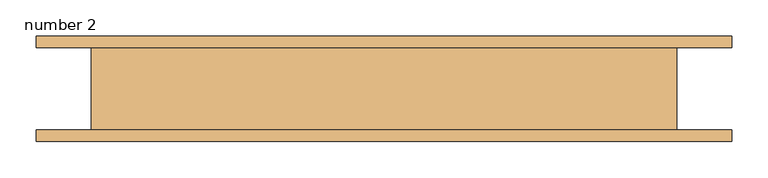
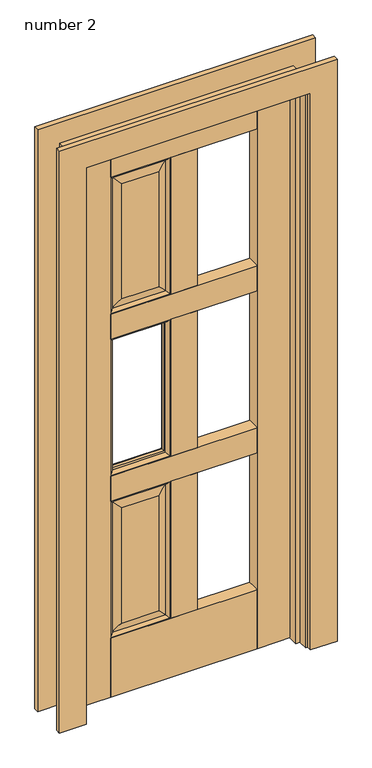
"""IFC4 building model written with IfcOpenShell, lengths in millimetres: door geometry, Door-Interior-Karona-K5660-6_Panel : number 2."""

from ifc_helpers import new_model, si_unit, frame, origin, origin_with_axes, place, context, project, spatial, polyline, ellipse_curve, outline, extrude, faceted_brep, source, transform, mapped, element, save
from ifc_brep_helpers import plane_surface, cylinder_surface, revolved_surface, advanced_brep


def number_2_7843cb6c(model_context):
    return source(origin(), model_context, "Body", "SolidModel", [
        advanced_brep(
        [(-254.0, 15.2908, 1311.275), (-242.6746863, 24.6126, 1299.9496863), (-57.3628137, 24.6126, 1299.9496863), (-46.0375, 15.2908, 1311.275), (-57.1627, 46.3324899, 1300.1498), (-48.2727, 54.4576, 1309.0398), (-48.2727, 54.4576, 811.8602), (-57.1627, 46.3324899, 820.7502), (-242.8748, 46.3324899, 820.7502), (-251.7648, 54.4576, 811.8602), (-251.7648, 54.4576, 1309.0398), (-242.8748, 46.3324899, 1300.1498), (-46.0375, 54.4576, 809.625), (-46.0375, 15.2908, 809.625), (-254.0, 15.2908, 809.625), (-254.0, 54.4576, 809.625), (-57.1627, 34.7218, 820.7502), (-242.8748, 34.7218, 820.7502), (-47.3075, 24.6126, 1310.005), (-47.3075, 34.7218, 1310.005), (-47.3075, 34.7218, 810.895), (-47.3075, 24.6126, 810.895), (-252.73, 24.6126, 810.895), (-252.73, 24.6126, 1310.005), (-57.3628137, 24.6126, 820.9503137), (-242.6746863, 24.6126, 820.9503137), (-252.73, 34.7218, 810.895), (-254.0, 54.4576, 1311.275), (-242.8748, 34.7218, 1300.1498), (-252.73, 34.7218, 1310.005), (-46.0375, 54.4576, 1311.275), (-57.1627, 34.7218, 1300.1498)],
        [
            (0, 1, ellipse_curve(frame((-252.9689876, 25.5788135, 1310.2439876), z_axis=(0.7071067811865475, 0.0, 0.7071067811865475), x_axis=(-0.7071067811865476, 0.0, 0.7071067811865474)), 14.6223259, 10.3395458)),
            (1, 2),
            (2, 3, ellipse_curve(frame((-47.0685124, 25.5788135, 1310.2439876), z_axis=(-0.7071067811865475, 0.0, 0.7071067811865475), x_axis=(-0.7071067811865476, 0.0, -0.7071067811865474)), 14.6223259, 10.3395458)),
            (3, 0),
            (4, 5, ellipse_curve(frame((-48.2727, 45.531597, 1309.0398), z_axis=(0.7071067811865475, 0.0, -0.7071067811865475), x_axis=(0.7071067811865474, 0.0, 0.7071067811865476)), 12.6232745, 8.926003)),
            (5, 6),
            (6, 7, ellipse_curve(frame((-48.2727, 45.531597, 811.8602), z_axis=(0.7071067811865475, 0.0, 0.7071067811865475), x_axis=(-0.7071067811865474, 0.0, 0.7071067811865476)), 12.6232745, 8.926003)),
            (7, 4),
            (8, 9, ellipse_curve(frame((-251.7648, 45.531597, 811.8602), z_axis=(-0.7071067811865475, 0.0, 0.7071067811865475), x_axis=(-0.7071067811865474, 0.0, -0.7071067811865476)), 12.6232745, 8.926003)),
            (9, 10),
            (10, 11, ellipse_curve(frame((-251.7648, 45.531597, 1309.0398), z_axis=(-0.7071067811865475, 0.0, -0.7071067811865475), x_axis=(0.7071067811865474, 0.0, -0.7071067811865476)), 12.6232745, 8.926003)),
            (11, 8),
            (12, 13),
            (13, 14),
            (14, 15),
            (15, 12),
            (16, 7),
            (7, 8),
            (8, 17),
            (17, 16),
            (18, 19),
            (19, 20),
            (20, 21),
            (21, 18),
            (22, 23),
            (23, 18),
            (21, 22),
            (24, 2),
            (1, 25),
            (25, 24),
            (13, 24, ellipse_curve(frame((-47.0685124, 25.5788135, 810.6560124), z_axis=(-0.7071067811865475, 0.0, -0.7071067811865475), x_axis=(0.7071067811865476, 0.0, -0.7071067811865474)), 14.6223259, 10.3395458)),
            (25, 14, ellipse_curve(frame((-252.9689876, 25.5788135, 810.6560124), z_axis=(0.7071067811865475, 0.0, -0.7071067811865475), x_axis=(0.7071067811865476, 0.0, 0.7071067811865474)), 14.6223259, 10.3395458)),
            (20, 26),
            (26, 22),
            (14, 0),
            (0, 27),
            (27, 15),
            (11, 28),
            (28, 17),
            (26, 29),
            (29, 23),
            (3, 30),
            (30, 27),
            (11, 4),
            (4, 31),
            (31, 28),
            (29, 19),
            (3, 13),
            (12, 30),
            (16, 31),
            (5, 10),
            (9, 6),
        ],
        [
            cylinder_surface(frame((-254.0, 25.5788135, 1310.2439876), z_axis=(-1.0, 0.0, 0.0), x_axis=(0.0, -1.0, 0.0)), 10.3395458),
            cylinder_surface(frame((-48.2727, 45.531597, 1311.275), z_axis=(0.0, 0.0, 1.0), x_axis=(0.0, -1.0, 0.0)), 8.926003),
            cylinder_surface(frame((-251.7648, 45.531597, 809.625), z_axis=(0.0, 0.0, -1.0), x_axis=(0.0, -1.0, 0.0)), 8.926003),
            plane_surface(frame((-46.0375, 15.2908, 809.625), z_axis=(0.0, 0.0, -1.0), x_axis=(-1.0, 0.0, 0.0))),
            plane_surface(frame((-57.1627, 46.3324899, 820.7502), z_axis=(0.0, 0.0, 1.0), x_axis=(-1.0, 0.0, 0.0))),
            plane_surface(frame((-47.3075, 34.7218, 1310.005), z_axis=(-1.0, 0.0, 0.0), x_axis=(0.0, 0.0, -1.0))),
            plane_surface(frame((-47.3075, 24.6126, 1310.005), z_axis=(0.0, 1.0, 0.0), x_axis=(0.0, 0.0, -1.0))),
            cylinder_surface(frame((-46.0375, 25.5788135, 810.6560124), z_axis=(1.0, 0.0, 0.0), x_axis=(0.0, -1.0, 0.0)), 10.3395458),
            plane_surface(frame((-47.3075, 34.7218, 810.895), z_axis=(0.0, 0.0, 1.0), x_axis=(-1.0, 0.0, 0.0))),
            plane_surface(frame((-254.0, 15.2908, 809.625), z_axis=(-1.0, 0.0, 0.0), x_axis=(0.0, 0.0, 1.0))),
            plane_surface(frame((-242.8748, 46.3324899, 820.7502), z_axis=(1.0, 0.0, 0.0), x_axis=(0.0, 0.0, 1.0))),
            plane_surface(frame((-252.73, 34.7218, 810.895), z_axis=(1.0, 0.0, 0.0), x_axis=(0.0, 0.0, 1.0))),
            plane_surface(frame((-254.0, 15.2908, 1311.275), z_axis=(0.0, 0.0, 1.0), x_axis=(1.0, 0.0, 0.0))),
            plane_surface(frame((-242.8748, 46.3324899, 1300.1498), z_axis=(0.0, 0.0, -1.0), x_axis=(1.0, 0.0, 0.0))),
            plane_surface(frame((-252.73, 34.7218, 1310.005), z_axis=(0.0, 0.0, -1.0), x_axis=(1.0, 0.0, 0.0))),
            plane_surface(frame((-46.0375, 15.2908, 1311.275), z_axis=(1.0, 0.0, 0.0), x_axis=(0.0, 0.0, -1.0))),
            plane_surface(frame((-57.1627, 46.3324899, 1300.1498), z_axis=(-1.0, 0.0, 0.0), x_axis=(0.0, 0.0, -1.0))),
            plane_surface(frame((-57.1627, 34.7218, 1300.1498), z_axis=(0.0, -1.0, 0.0), x_axis=(0.0, 0.0, -1.0))),
            plane_surface(frame((-46.0375, 54.4576, 1311.275), z_axis=(0.0, 1.0, 0.0), x_axis=(0.0, 0.0, -1.0))),
            cylinder_surface(frame((-46.0375, 45.531597, 811.8602), z_axis=(1.0, 0.0, 0.0), x_axis=(0.0, -1.0, 0.0)), 8.926003),
            cylinder_surface(frame((-252.9689876, 25.5788135, 809.625), z_axis=(0.0, 0.0, -1.0), x_axis=(0.0, -1.0, 0.0)), 10.3395458),
            cylinder_surface(frame((-254.0, 45.531597, 1309.0398), z_axis=(-1.0, 0.0, 0.0), x_axis=(0.0, -1.0, 0.0)), 8.926003),
            cylinder_surface(frame((-47.0685124, 25.5788135, 1311.275), z_axis=(0.0, 0.0, 1.0), x_axis=(0.0, -1.0, 0.0)), 10.3395458),
        ],
        [
            (0, [[1, 2, 3, 4]]),
            (1, [[5, 6, 7, 8]]),
            (2, [[9, 10, 11, 12]]),
            (3, [[13, 14, 15, 16]]),
            (4, [[17, 18, 19, 20]]),
            (5, [[21, 22, 23, 24]]),
            (6, [[25, 26, -24, 27], [28, -2, 29, 30]]),
            (7, [[31, -30, 32, -14]]),
            (8, [[-23, 33, 34, -27]]),
            (9, [[-15, 35, 36, 37]]),
            (10, [[-19, -12, 38, 39]]),
            (11, [[-34, 40, 41, -25]]),
            (12, [[-36, -4, 42, 43]]),
            (13, [[-38, 44, 45, 46]]),
            (14, [[-41, 47, -21, -26]]),
            (15, [[-42, 48, -13, 49]]),
            (16, [[-45, -8, -17, 50]]),
            (17, [[-22, -47, -40, -33], [-39, -46, -50, -20]]),
            (18, [[-37, -43, -49, -16], [-6, 51, -10, 52]]),
            (19, [[-7, -52, -9, -18]]),
            (20, [[-32, -29, -1, -35]]),
            (21, [[-11, -51, -5, -44]]),
            (22, [[-3, -28, -31, -48]]),
        ],
    ),
        advanced_brep(
        [(-242.8748, 54.4576, 1893.8748), (-57.1627, 54.4576, 1893.8748), (-57.1627, 54.4576, 1414.4752), (-242.8748, 54.4576, 1414.4752), (-242.8748, 34.7218, 1893.8748), (-57.1627, 34.7218, 1893.8748), (-57.1627, 36.0454899, 1893.8748), (-242.8748, 36.0454899, 1893.8748), (-242.8748, 44.5515929, 1893.8748), (-57.1627, 44.5515929, 1893.8748), (-57.1627, 34.7218, 1414.4752), (-242.8748, 34.7218, 1414.4752), (-242.8748, 36.0454899, 1414.4752), (-57.1627, 36.0454899, 1414.4752), (-57.1627, 44.5515929, 1414.4752), (-242.8748, 44.5515929, 1414.4752), (-87.1686653, 44.5515929, 1863.8688347), (-212.8688347, 44.5515929, 1863.8688347), (-87.1686653, 44.5515929, 1444.4811653), (-212.8688347, 44.5515929, 1444.4811653)],
        [
            (0, 1),
            (1, 2),
            (2, 3),
            (3, 0),
            (4, 5),
            (5, 6),
            (6, 7),
            (7, 4),
            (0, 8),
            (8, 9),
            (9, 1),
            (10, 11),
            (11, 12),
            (12, 13),
            (13, 10),
            (2, 14),
            (14, 15),
            (15, 3),
            (15, 8),
            (11, 4),
            (7, 12),
            (9, 14),
            (5, 10),
            (13, 6),
            (16, 17),
            (17, 7, ellipse_curve(frame((-244.8131685, 100.0605261, 1895.8131685), z_axis=(-0.7071067811865475, 0.0, -0.7071067811865475), x_axis=(-0.7071067811865476, 0.0, 0.7071067811865474)), 90.5724254, 64.0443762)),
            (6, 16, ellipse_curve(frame((-55.2243315, 100.0605261, 1895.8131685), z_axis=(0.7071067811865475, 0.0, -0.7071067811865475), x_axis=(-0.7071067811865476, 0.0, -0.7071067811865474)), 90.5724254, 64.0443762)),
            (18, 16),
            (13, 18, ellipse_curve(frame((-55.2243315, 100.0605261, 1412.5368315), z_axis=(-0.7071067811865475, 0.0, -0.7071067811865475), x_axis=(-0.7071067811865474, 0.0, 0.7071067811865476)), 90.5724254, 64.0443762)),
            (19, 18),
            (12, 19, ellipse_curve(frame((-244.8131685, 100.0605261, 1412.5368315), z_axis=(-0.7071067811865475, 0.0, 0.7071067811865475), x_axis=(0.7071067811865476, 0.0, 0.7071067811865474)), 90.5724254, 64.0443762)),
            (17, 19),
        ],
        [
            plane_surface(frame((-57.1627, 54.4576, 1893.8748), z_axis=(0.0, 1.0, 0.0), x_axis=(0.0, 0.0, -1.0))),
            plane_surface(frame((-57.1627, 34.7218, 1893.8748), z_axis=(0.0, 0.0, 1.0), x_axis=(1.0, 0.0, 0.0))),
            plane_surface(frame((-57.1627, 34.7218, 1414.4752), z_axis=(0.0, 0.0, -1.0), x_axis=(-1.0, 0.0, 0.0))),
            plane_surface(frame((-242.8748, 54.4576, 1893.8748), z_axis=(-1.0, 0.0, 0.0), x_axis=(0.0, 0.0, -1.0))),
            plane_surface(frame((-57.1627, 34.7218, 1893.8748), z_axis=(1.0, 0.0, 0.0), x_axis=(0.0, 0.0, -1.0))),
            plane_surface(frame((-242.8748, 34.7218, 1893.8748), z_axis=(0.0, -1.0, 0.0), x_axis=(0.0, 0.0, -1.0))),
            revolved_surface(polyline([(-308.8575446888527, 100.0605261, 1831.7687923), (8.820044688852704, 100.0605261, 1831.7687923)]), (-254.0, 100.0605261, 1895.8131685), (-1.0, 0.0, 0.0)),
            revolved_surface(polyline([(-119.2687077, 100.0605261, 1959.8575446888528), (-119.2687077, 100.0605261, 1348.4924553111473)]), (-55.2243315, 100.0605261, 1905.0), (0.0, 0.0, 1.0)),
            revolved_surface(polyline([(8.820044688852683, 100.0605261, 1476.5812077), (-308.8575446888527, 100.0605261, 1476.5812077)]), (-46.0375, 100.0605261, 1412.5368315), (1.0, 0.0, 0.0)),
            revolved_surface(polyline([(-180.76879229999997, 100.0605261, 1348.4924553111473), (-180.76879229999997, 100.0605261, 1959.8575446888526)]), (-244.8131685, 100.0605261, 1403.35), (0.0, 0.0, -1.0)),
            plane_surface(frame((-254.0, 44.5515929, 1403.35), z_axis=(0.0, -1.0, 0.0), x_axis=(0.0, 0.0, 1.0))),
        ],
        [
            (0, [[1, 2, 3, 4]]),
            (1, [[5, 6, 7, 8]]),
            (1, [[-1, 9, 10, 11]]),
            (2, [[12, 13, 14, 15]]),
            (2, [[-3, 16, 17, 18]]),
            (3, [[-4, -18, 19, -9]]),
            (3, [[20, -8, 21, -13]]),
            (4, [[-2, -11, 22, -16]]),
            (4, [[23, -15, 24, -6]]),
            (5, [[-5, -20, -12, -23]]),
            (6, [[25, 26, -7, 27]]),
            (7, [[28, -27, -24, 29]]),
            (8, [[30, -29, -14, 31]]),
            (9, [[32, -31, -21, -26]]),
            (10, [[-10, -19, -17, -22], [-25, -28, -30, -32]]),
        ],
    ),
        advanced_brep(
        [(-242.8748, 24.6126, 1893.8748), (-57.1627, 24.6126, 1893.8748), (-57.1627, 24.6126, 1414.4752), (-242.8748, 24.6126, 1414.4752), (-214.0448579, 15.4432, 1443.3051421), (-85.9926421, 15.4432, 1443.3051421), (-85.9926421, 15.4432, 1865.0448579), (-214.0448579, 15.4432, 1865.0448579), (-242.8748, 23.2889101, 1893.8748), (-57.1627, 23.2889101, 1893.8748), (-57.1627, 23.2889101, 1414.4752), (-242.8748, 23.2889101, 1414.4752)],
        [
            (0, 1),
            (1, 2),
            (2, 3),
            (3, 0),
            (4, 5),
            (5, 6),
            (6, 7),
            (7, 4),
            (0, 8),
            (8, 9),
            (9, 1),
            (2, 10),
            (10, 11),
            (11, 3),
            (4, 11, ellipse_curve(frame((-244.8131685, -40.7261261, 1412.5368315), z_axis=(-0.7071067811865475, 0.0, 0.7071067811865475), x_axis=(0.7071067811865476, 0.0, 0.7071067811865474)), 90.5724254, 64.0443762)),
            (10, 5, ellipse_curve(frame((-55.2243315, -40.7261261, 1412.5368315), z_axis=(0.7071067811865475, 0.0, 0.7071067811865475), x_axis=(0.7071067811865476, 0.0, -0.7071067811865474)), 90.5724254, 64.0443762)),
            (7, 8, ellipse_curve(frame((-244.8131685, -40.7261261, 1895.8131685), z_axis=(0.7071067811865475, 0.0, 0.7071067811865475), x_axis=(0.7071067811865474, 0.0, -0.7071067811865476)), 90.5724254, 64.0443762)),
            (8, 11),
            (6, 9, ellipse_curve(frame((-55.2243315, -40.7261261, 1895.8131685), z_axis=(0.7071067811865475, 0.0, -0.7071067811865475), x_axis=(-0.7071067811865476, 0.0, -0.7071067811865474)), 90.5724254, 64.0443762)),
            (10, 9),
        ],
        [
            plane_surface(frame((-57.1627, 24.6126, 1893.8748), z_axis=(0.0, 1.0, 0.0), x_axis=(0.0, 0.0, -1.0))),
            plane_surface(frame((-242.8748, 15.4432, 1893.8748), z_axis=(0.0, -1.0, 0.0), x_axis=(0.0, 0.0, -1.0))),
            plane_surface(frame((-57.1627, 34.7218, 1893.8748), z_axis=(0.0, 0.0, 1.0), x_axis=(1.0, 0.0, 0.0))),
            plane_surface(frame((-57.1627, 34.7218, 1414.4752), z_axis=(0.0, 0.0, -1.0), x_axis=(-1.0, 0.0, 0.0))),
            revolved_surface(polyline([(8.820044688852711, -40.7261261, 1476.5812077), (-308.8575446888527, -40.7261261, 1476.5812077)]), (-46.0375, -40.7261261, 1412.5368315), (1.0, 0.0, 0.0)),
            revolved_surface(polyline([(-180.76879229999997, -40.7261261, 1348.4924553111473), (-180.76879229999997, -40.7261261, 1959.8575446888528)]), (-244.8131685, -40.7261261, 1403.35), (0.0, 0.0, -1.0)),
            revolved_surface(polyline([(-308.85754468885267, -40.7261261, 1831.7687923), (8.820044688852704, -40.7261261, 1831.7687923)]), (-254.0, -40.7261261, 1895.8131685), (-1.0, 0.0, 0.0)),
            revolved_surface(polyline([(-119.2687077, -40.7261261, 1959.8575446888528), (-119.2687077, -40.7261261, 1348.4924553111473)]), (-55.2243315, -40.7261261, 1905.0), (0.0, 0.0, 1.0)),
            plane_surface(frame((-242.8748, 24.6126, 1893.8748), z_axis=(-1.0, 0.0, 0.0), x_axis=(0.0, 0.0, -1.0))),
            plane_surface(frame((-57.1627, 15.4432, 1893.8748), z_axis=(1.0, 0.0, 0.0), x_axis=(0.0, 0.0, -1.0))),
        ],
        [
            (0, [[1, 2, 3, 4]]),
            (1, [[5, 6, 7, 8]]),
            (2, [[-1, 9, 10, 11]]),
            (3, [[-3, 12, 13, 14]]),
            (4, [[15, -13, 16, -5]]),
            (5, [[-15, -8, 17, 18]]),
            (6, [[-17, -7, 19, -10]]),
            (7, [[-19, -6, -16, 20]]),
            (8, [[-4, -14, -18, -9]]),
            (9, [[-2, -11, -20, -12]]),
        ],
    ),
        advanced_brep(
        [(-254.0, 15.2908, 1905.0), (-242.6746863, 24.6126, 1893.6746863), (-57.3628137, 24.6126, 1893.6746863), (-46.0375, 15.2908, 1905.0), (-57.1627, 46.3324899, 1893.8748), (-48.2727, 54.4576, 1902.7648), (-48.2727, 54.4576, 1405.5852), (-57.1627, 46.3324899, 1414.4752), (-242.8748, 46.3324899, 1414.4752), (-251.7648, 54.4576, 1405.5852), (-251.7648, 54.4576, 1902.7648), (-242.8748, 46.3324899, 1893.8748), (-46.0375, 54.4576, 1403.35), (-46.0375, 15.2908, 1403.35), (-254.0, 15.2908, 1403.35), (-254.0, 54.4576, 1403.35), (-57.1627, 34.7218, 1414.4752), (-242.8748, 34.7218, 1414.4752), (-47.3075, 24.6126, 1903.73), (-47.3075, 34.7218, 1903.73), (-47.3075, 34.7218, 1404.62), (-47.3075, 24.6126, 1404.62), (-252.73, 24.6126, 1404.62), (-252.73, 24.6126, 1903.73), (-57.3628137, 24.6126, 1414.6753137), (-242.6746863, 24.6126, 1414.6753137), (-252.73, 34.7218, 1404.62), (-254.0, 54.4576, 1905.0), (-242.8748, 34.7218, 1893.8748), (-252.73, 34.7218, 1903.73), (-46.0375, 54.4576, 1905.0), (-57.1627, 34.7218, 1893.8748)],
        [
            (0, 1, ellipse_curve(frame((-252.9689876, 25.5788135, 1903.9689876), z_axis=(0.7071067811865475, 0.0, 0.7071067811865475), x_axis=(-0.7071067811865476, 0.0, 0.7071067811865474)), 14.6223259, 10.3395458)),
            (1, 2),
            (2, 3, ellipse_curve(frame((-47.0685124, 25.5788135, 1903.9689876), z_axis=(-0.7071067811865475, 0.0, 0.7071067811865475), x_axis=(-0.7071067811865476, 0.0, -0.7071067811865474)), 14.6223259, 10.3395458)),
            (3, 0),
            (4, 5, ellipse_curve(frame((-48.2727, 45.531597, 1902.7648), z_axis=(0.7071067811865475, 0.0, -0.7071067811865475), x_axis=(0.7071067811865474, 0.0, 0.7071067811865476)), 12.6232745, 8.926003)),
            (5, 6),
            (6, 7, ellipse_curve(frame((-48.2727, 45.531597, 1405.5852), z_axis=(0.7071067811865475, 0.0, 0.7071067811865475), x_axis=(-0.7071067811865474, 0.0, 0.7071067811865476)), 12.6232745, 8.926003)),
            (7, 4),
            (8, 9, ellipse_curve(frame((-251.7648, 45.531597, 1405.5852), z_axis=(-0.7071067811865475, 0.0, 0.7071067811865475), x_axis=(-0.7071067811865474, 0.0, -0.7071067811865476)), 12.6232745, 8.926003)),
            (9, 10),
            (10, 11, ellipse_curve(frame((-251.7648, 45.531597, 1902.7648), z_axis=(-0.7071067811865475, 0.0, -0.7071067811865475), x_axis=(0.7071067811865474, 0.0, -0.7071067811865476)), 12.6232745, 8.926003)),
            (11, 8),
            (12, 13),
            (13, 14),
            (14, 15),
            (15, 12),
            (16, 7),
            (7, 8),
            (8, 17),
            (17, 16),
            (18, 19),
            (19, 20),
            (20, 21),
            (21, 18),
            (22, 23),
            (23, 18),
            (21, 22),
            (24, 2),
            (1, 25),
            (25, 24),
            (13, 24, ellipse_curve(frame((-47.0685124, 25.5788135, 1404.3810124), z_axis=(-0.7071067811865475, 0.0, -0.7071067811865475), x_axis=(0.7071067811865476, 0.0, -0.7071067811865474)), 14.6223259, 10.3395458)),
            (25, 14, ellipse_curve(frame((-252.9689876, 25.5788135, 1404.3810124), z_axis=(0.7071067811865475, 0.0, -0.7071067811865475), x_axis=(0.7071067811865476, 0.0, 0.7071067811865474)), 14.6223259, 10.3395458)),
            (20, 26),
            (26, 22),
            (14, 0),
            (0, 27),
            (27, 15),
            (11, 28),
            (28, 17),
            (26, 29),
            (29, 23),
            (3, 30),
            (30, 27),
            (11, 4),
            (4, 31),
            (31, 28),
            (29, 19),
            (3, 13),
            (12, 30),
            (16, 31),
            (5, 10),
            (9, 6),
        ],
        [
            cylinder_surface(frame((-254.0, 25.5788135, 1903.9689876), z_axis=(-1.0, 0.0, 0.0), x_axis=(0.0, -1.0, 0.0)), 10.3395458),
            cylinder_surface(frame((-48.2727, 45.531597, 1905.0), z_axis=(0.0, 0.0, 1.0), x_axis=(0.0, -1.0, 0.0)), 8.926003),
            cylinder_surface(frame((-251.7648, 45.531597, 1403.35), z_axis=(0.0, 0.0, -1.0), x_axis=(0.0, -1.0, 0.0)), 8.926003),
            plane_surface(frame((-46.0375, 15.2908, 1403.35), z_axis=(0.0, 0.0, -1.0), x_axis=(-1.0, 0.0, 0.0))),
            plane_surface(frame((-57.1627, 46.3324899, 1414.4752), z_axis=(0.0, 0.0, 1.0), x_axis=(-1.0, 0.0, 0.0))),
            plane_surface(frame((-47.3075, 34.7218, 1903.73), z_axis=(-1.0, 0.0, 0.0), x_axis=(0.0, 0.0, -1.0))),
            plane_surface(frame((-47.3075, 24.6126, 1903.73), z_axis=(0.0, 1.0, 0.0), x_axis=(0.0, 0.0, -1.0))),
            cylinder_surface(frame((-46.0375, 25.5788135, 1404.3810124), z_axis=(1.0, 0.0, 0.0), x_axis=(0.0, -1.0, 0.0)), 10.3395458),
            plane_surface(frame((-47.3075, 34.7218, 1404.62), z_axis=(0.0, 0.0, 1.0), x_axis=(-1.0, 0.0, 0.0))),
            plane_surface(frame((-254.0, 15.2908, 1403.35), z_axis=(-1.0, 0.0, 0.0), x_axis=(0.0, 0.0, 1.0))),
            plane_surface(frame((-242.8748, 46.3324899, 1414.4752), z_axis=(1.0, 0.0, 0.0), x_axis=(0.0, 0.0, 1.0))),
            plane_surface(frame((-252.73, 34.7218, 1404.62), z_axis=(1.0, 0.0, 0.0), x_axis=(0.0, 0.0, 1.0))),
            plane_surface(frame((-254.0, 15.2908, 1905.0), z_axis=(0.0, 0.0, 1.0), x_axis=(1.0, 0.0, 0.0))),
            plane_surface(frame((-242.8748, 46.3324899, 1893.8748), z_axis=(0.0, 0.0, -1.0), x_axis=(1.0, 0.0, 0.0))),
            plane_surface(frame((-252.73, 34.7218, 1903.73), z_axis=(0.0, 0.0, -1.0), x_axis=(1.0, 0.0, 0.0))),
            plane_surface(frame((-46.0375, 15.2908, 1905.0), z_axis=(1.0, 0.0, 0.0), x_axis=(0.0, 0.0, -1.0))),
            plane_surface(frame((-57.1627, 46.3324899, 1893.8748), z_axis=(-1.0, 0.0, 0.0), x_axis=(0.0, 0.0, -1.0))),
            plane_surface(frame((-57.1627, 34.7218, 1893.8748), z_axis=(0.0, -1.0, 0.0), x_axis=(0.0, 0.0, -1.0))),
            plane_surface(frame((-46.0375, 54.4576, 1905.0), z_axis=(0.0, 1.0, 0.0), x_axis=(0.0, 0.0, -1.0))),
            cylinder_surface(frame((-46.0375, 45.531597, 1405.5852), z_axis=(1.0, 0.0, 0.0), x_axis=(0.0, -1.0, 0.0)), 8.926003),
            cylinder_surface(frame((-252.9689876, 25.5788135, 1403.35), z_axis=(0.0, 0.0, -1.0), x_axis=(0.0, -1.0, 0.0)), 10.3395458),
            cylinder_surface(frame((-254.0, 45.531597, 1902.7648), z_axis=(-1.0, 0.0, 0.0), x_axis=(0.0, -1.0, 0.0)), 8.926003),
            cylinder_surface(frame((-47.0685124, 25.5788135, 1905.0), z_axis=(0.0, 0.0, 1.0), x_axis=(0.0, -1.0, 0.0)), 10.3395458),
        ],
        [
            (0, [[1, 2, 3, 4]]),
            (1, [[5, 6, 7, 8]]),
            (2, [[9, 10, 11, 12]]),
            (3, [[13, 14, 15, 16]]),
            (4, [[17, 18, 19, 20]]),
            (5, [[21, 22, 23, 24]]),
            (6, [[25, 26, -24, 27], [28, -2, 29, 30]]),
            (7, [[31, -30, 32, -14]]),
            (8, [[-23, 33, 34, -27]]),
            (9, [[-15, 35, 36, 37]]),
            (10, [[-19, -12, 38, 39]]),
            (11, [[-34, 40, 41, -25]]),
            (12, [[-36, -4, 42, 43]]),
            (13, [[-38, 44, 45, 46]]),
            (14, [[-41, 47, -21, -26]]),
            (15, [[-42, 48, -13, 49]]),
            (16, [[-45, -8, -17, 50]]),
            (17, [[-22, -47, -40, -33], [-39, -46, -50, -20]]),
            (18, [[-37, -43, -49, -16], [-6, 51, -10, 52]]),
            (19, [[-7, -52, -9, -18]]),
            (20, [[-32, -29, -1, -35]]),
            (21, [[-11, -51, -5, -44]]),
            (22, [[-3, -28, -31, -48]]),
        ],
    ),
        advanced_brep(
        [(-242.8748, 34.7218, 706.4248), (-57.1627, 34.7218, 706.4248), (-57.1627, 36.0454899, 706.4248), (-242.8748, 36.0454899, 706.4248), (-57.1627, 54.4576, 706.4248), (-242.8748, 54.4576, 706.4248), (-242.8748, 44.5515929, 706.4248), (-57.1627, 44.5515929, 706.4248), (-57.1627, 34.7218, 227.0252), (-242.8748, 34.7218, 227.0252), (-242.8748, 36.0454899, 227.0252), (-57.1627, 36.0454899, 227.0252), (-242.8748, 54.4576, 227.0252), (-57.1627, 54.4576, 227.0252), (-57.1627, 44.5515929, 227.0252), (-242.8748, 44.5515929, 227.0252), (-87.1686653, 44.5515929, 676.4188347), (-212.8688347, 44.5515929, 676.4188347), (-87.1686653, 44.5515929, 257.0311653), (-212.8688347, 44.5515929, 257.0311653)],
        [
            (0, 1),
            (1, 2),
            (2, 3),
            (3, 0),
            (4, 5),
            (5, 6),
            (6, 7),
            (7, 4),
            (8, 9),
            (9, 10),
            (10, 11),
            (11, 8),
            (12, 13),
            (13, 14),
            (14, 15),
            (15, 12),
            (5, 12),
            (15, 6),
            (9, 0),
            (3, 10),
            (4, 13),
            (7, 14),
            (1, 8),
            (11, 2),
            (16, 17),
            (17, 3, ellipse_curve(frame((-244.8131685, 100.0605261, 708.3631685), z_axis=(-0.7071067811865475, 0.0, -0.7071067811865475), x_axis=(-0.7071067811865476, 0.0, 0.7071067811865474)), 90.5724254, 64.0443762)),
            (2, 16, ellipse_curve(frame((-55.2243315, 100.0605261, 708.3631685), z_axis=(0.7071067811865475, 0.0, -0.7071067811865475), x_axis=(-0.7071067811865476, 0.0, -0.7071067811865474)), 90.5724254, 64.0443762)),
            (18, 16),
            (11, 18, ellipse_curve(frame((-55.2243315, 100.0605261, 225.0868315), z_axis=(-0.7071067811865475, 0.0, -0.7071067811865475), x_axis=(-0.7071067811865474, 0.0, 0.7071067811865476)), 90.5724254, 64.0443762)),
            (19, 18),
            (10, 19, ellipse_curve(frame((-244.8131685, 100.0605261, 225.0868315), z_axis=(-0.7071067811865475, 0.0, 0.7071067811865475), x_axis=(0.7071067811865476, 0.0, 0.7071067811865474)), 90.5724254, 64.0443762)),
            (17, 19),
        ],
        [
            plane_surface(frame((-57.1627, 34.7218, 706.4248), z_axis=(0.0, 0.0, 1.0), x_axis=(1.0, 0.0, 0.0))),
            plane_surface(frame((-57.1627, 34.7218, 227.0252), z_axis=(0.0, 0.0, -1.0), x_axis=(-1.0, 0.0, 0.0))),
            plane_surface(frame((-242.8748, 54.4576, 706.4248), z_axis=(-1.0, 0.0, 0.0), x_axis=(0.0, 0.0, -1.0))),
            plane_surface(frame((-57.1627, 54.4576, 706.4248), z_axis=(0.0, 1.0, 0.0), x_axis=(0.0, 0.0, -1.0))),
            plane_surface(frame((-57.1627, 34.7218, 706.4248), z_axis=(1.0, 0.0, 0.0), x_axis=(0.0, 0.0, -1.0))),
            plane_surface(frame((-242.8748, 34.7218, 706.4248), z_axis=(0.0, -1.0, 0.0), x_axis=(0.0, 0.0, -1.0))),
            revolved_surface(polyline([(-308.8575446888527, 100.0605261, 644.3187923), (8.820044688852704, 100.0605261, 644.3187923)]), (-254.0, 100.0605261, 708.3631685), (-1.0, 0.0, 0.0)),
            revolved_surface(polyline([(-119.2687077, 100.0605261, 772.4075446888527), (-119.2687077, 100.0605261, 161.04245531114725)]), (-55.2243315, 100.0605261, 717.55), (0.0, 0.0, 1.0)),
            revolved_surface(polyline([(8.820044688852683, 100.0605261, 289.1312077), (-308.8575446888527, 100.0605261, 289.1312077)]), (-46.0375, 100.0605261, 225.0868315), (1.0, 0.0, 0.0)),
            revolved_surface(polyline([(-180.76879229999997, 100.0605261, 161.0424553111473), (-180.76879229999997, 100.0605261, 772.4075446888527)]), (-244.8131685, 100.0605261, 215.9), (0.0, 0.0, -1.0)),
            plane_surface(frame((-254.0, 44.5515929, 215.9), z_axis=(0.0, -1.0, 0.0), x_axis=(0.0, 0.0, 1.0))),
        ],
        [
            (0, [[1, 2, 3, 4]]),
            (0, [[5, 6, 7, 8]]),
            (1, [[9, 10, 11, 12]]),
            (1, [[13, 14, 15, 16]]),
            (2, [[17, -16, 18, -6]]),
            (2, [[19, -4, 20, -10]]),
            (3, [[-5, 21, -13, -17]]),
            (4, [[-21, -8, 22, -14]]),
            (4, [[23, -12, 24, -2]]),
            (5, [[-1, -19, -9, -23]]),
            (6, [[25, 26, -3, 27]]),
            (7, [[28, -27, -24, 29]]),
            (8, [[30, -29, -11, 31]]),
            (9, [[32, -31, -20, -26]]),
            (10, [[-7, -18, -15, -22], [-25, -28, -30, -32]]),
        ],
    ),
        advanced_brep(
        [(-57.1627, 24.6126, 706.4248), (-242.8748, 24.6126, 706.4248), (-242.8748, 23.2889101, 706.4248), (-57.1627, 23.2889101, 706.4248), (-242.8748, 24.6126, 227.0252), (-57.1627, 24.6126, 227.0252), (-57.1627, 23.2889101, 227.0252), (-242.8748, 23.2889101, 227.0252), (-214.0448579, 15.4432, 255.8551421), (-85.9926421, 15.4432, 255.8551421), (-85.9926421, 15.4432, 677.5948579), (-214.0448579, 15.4432, 677.5948579)],
        [
            (0, 1),
            (1, 2),
            (2, 3),
            (3, 0),
            (4, 5),
            (5, 6),
            (6, 7),
            (7, 4),
            (0, 5),
            (4, 1),
            (8, 9),
            (9, 10),
            (10, 11),
            (11, 8),
            (8, 7, ellipse_curve(frame((-244.8131685, -40.7261261, 225.0868315), z_axis=(-0.7071067811865475, 0.0, 0.7071067811865475), x_axis=(0.7071067811865476, 0.0, 0.7071067811865474)), 90.5724254, 64.0443762)),
            (6, 9, ellipse_curve(frame((-55.2243315, -40.7261261, 225.0868315), z_axis=(0.7071067811865475, 0.0, 0.7071067811865475), x_axis=(0.7071067811865476, 0.0, -0.7071067811865474)), 90.5724254, 64.0443762)),
            (11, 2, ellipse_curve(frame((-244.8131685, -40.7261261, 708.3631685), z_axis=(0.7071067811865475, 0.0, 0.7071067811865475), x_axis=(0.7071067811865474, 0.0, -0.7071067811865476)), 90.5724254, 64.0443762)),
            (2, 7),
            (10, 3, ellipse_curve(frame((-55.2243315, -40.7261261, 708.3631685), z_axis=(0.7071067811865475, 0.0, -0.7071067811865475), x_axis=(-0.7071067811865476, 0.0, -0.7071067811865474)), 90.5724254, 64.0443762)),
            (6, 3),
        ],
        [
            plane_surface(frame((-57.1627, 34.7218, 706.4248), z_axis=(0.0, 0.0, 1.0), x_axis=(1.0, 0.0, 0.0))),
            plane_surface(frame((-57.1627, 34.7218, 227.0252), z_axis=(0.0, 0.0, -1.0), x_axis=(-1.0, 0.0, 0.0))),
            plane_surface(frame((-57.1627, 24.6126, 706.4248), z_axis=(0.0, 1.0, 0.0), x_axis=(0.0, 0.0, -1.0))),
            plane_surface(frame((-242.8748, 15.4432, 706.4248), z_axis=(0.0, -1.0, 0.0), x_axis=(0.0, 0.0, -1.0))),
            revolved_surface(polyline([(8.820044688852711, -40.7261261, 289.1312077), (-308.8575446888527, -40.7261261, 289.1312077)]), (-46.0375, -40.7261261, 225.0868315), (1.0, 0.0, 0.0)),
            revolved_surface(polyline([(-180.76879229999997, -40.7261261, 161.0424553111473), (-180.76879229999997, -40.7261261, 772.4075446888527)]), (-244.8131685, -40.7261261, 215.9), (0.0, 0.0, -1.0)),
            revolved_surface(polyline([(-308.85754468885267, -40.7261261, 644.3187923), (8.820044688852704, -40.7261261, 644.3187923)]), (-254.0, -40.7261261, 708.3631685), (-1.0, 0.0, 0.0)),
            revolved_surface(polyline([(-119.2687077, -40.7261261, 772.4075446888527), (-119.2687077, -40.7261261, 161.04245531114736)]), (-55.2243315, -40.7261261, 717.55), (0.0, 0.0, 1.0)),
            plane_surface(frame((-242.8748, 24.6126, 706.4248), z_axis=(-1.0, 0.0, 0.0), x_axis=(0.0, 0.0, -1.0))),
            plane_surface(frame((-57.1627, 15.4432, 706.4248), z_axis=(1.0, 0.0, 0.0), x_axis=(0.0, 0.0, -1.0))),
        ],
        [
            (0, [[1, 2, 3, 4]]),
            (1, [[5, 6, 7, 8]]),
            (2, [[-1, 9, -5, 10]]),
            (3, [[11, 12, 13, 14]]),
            (4, [[15, -7, 16, -11]]),
            (5, [[-15, -14, 17, 18]]),
            (6, [[-17, -13, 19, -3]]),
            (7, [[-19, -12, -16, 20]]),
            (8, [[-10, -8, -18, -2]]),
            (9, [[-9, -4, -20, -6]]),
        ],
    ),
        advanced_brep(
        [(-254.0, 15.2908, 717.55), (-242.6746863, 24.6126, 706.2246863), (-57.3628137, 24.6126, 706.2246863), (-46.0375, 15.2908, 717.55), (-57.1627, 46.3324899, 706.4248), (-48.2727, 54.4576, 715.3148), (-48.2727, 54.4576, 218.1352), (-57.1627, 46.3324899, 227.0252), (-254.0, 54.4576, 215.9), (-254.0, 54.4576, 717.55), (-46.0375, 54.4576, 717.55), (-46.0375, 54.4576, 215.9), (-251.7648, 54.4576, 715.3148), (-251.7648, 54.4576, 218.1352), (-46.0375, 15.2908, 215.9), (-254.0, 15.2908, 215.9), (-57.1627, 34.7218, 227.0252), (-242.8748, 46.3324899, 227.0252), (-242.8748, 34.7218, 227.0252), (-47.3075, 24.6126, 217.17), (-47.3075, 34.7218, 217.17), (-252.73, 34.7218, 217.17), (-252.73, 24.6126, 217.17), (-242.8748, 46.3324899, 706.4248), (-242.8748, 34.7218, 706.4248), (-252.73, 34.7218, 716.28), (-252.73, 24.6126, 716.28), (-57.1627, 34.7218, 706.4248), (-47.3075, 34.7218, 716.28), (-47.3075, 24.6126, 716.28), (-57.3628137, 24.6126, 227.2253137), (-242.6746863, 24.6126, 227.2253137)],
        [
            (0, 1, ellipse_curve(frame((-252.9689876, 25.5788135, 716.5189876), z_axis=(0.7071067811865475, 0.0, 0.7071067811865475), x_axis=(-0.7071067811865476, 0.0, 0.7071067811865474)), 14.6223259, 10.3395458)),
            (1, 2),
            (2, 3, ellipse_curve(frame((-47.0685124, 25.5788135, 716.5189876), z_axis=(-0.7071067811865475, 0.0, 0.7071067811865475), x_axis=(-0.7071067811865476, 0.0, -0.7071067811865474)), 14.6223259, 10.3395458)),
            (3, 0),
            (4, 5, ellipse_curve(frame((-48.2727, 45.531597, 715.3148), z_axis=(0.7071067811865475, 0.0, -0.7071067811865475), x_axis=(0.7071067811865474, 0.0, 0.7071067811865476)), 12.6232745, 8.926003)),
            (5, 6),
            (6, 7, ellipse_curve(frame((-48.2727, 45.531597, 218.1352), z_axis=(0.7071067811865475, 0.0, 0.7071067811865475), x_axis=(-0.7071067811865474, 0.0, 0.7071067811865476)), 12.6232745, 8.926003)),
            (7, 4),
            (8, 9),
            (9, 10),
            (10, 11),
            (11, 8),
            (5, 12),
            (12, 13),
            (13, 6),
            (11, 14),
            (14, 15),
            (15, 8),
            (16, 7),
            (7, 17),
            (17, 18),
            (18, 16),
            (19, 20),
            (20, 21),
            (21, 22),
            (22, 19),
            (15, 0),
            (0, 9),
            (17, 23),
            (23, 24),
            (24, 18),
            (21, 25),
            (25, 26),
            (26, 22),
            (3, 10),
            (23, 4),
            (4, 27),
            (27, 24),
            (25, 28),
            (28, 29),
            (29, 26),
            (3, 14),
            (16, 27),
            (20, 28),
            (19, 29),
            (30, 2),
            (1, 31),
            (31, 30),
            (30, 14, ellipse_curve(frame((-47.0685124, 25.5788135, 216.9310124), z_axis=(0.7071067811865475, 0.0, 0.7071067811865475), x_axis=(-0.7071067811865474, 0.0, 0.7071067811865476)), 14.6223259, 10.3395458)),
            (17, 13, ellipse_curve(frame((-251.7648, 45.531597, 218.1352), z_axis=(-0.7071067811865475, 0.0, 0.7071067811865475), x_axis=(-0.7071067811865474, 0.0, -0.7071067811865476)), 12.6232745, 8.926003)),
            (12, 23, ellipse_curve(frame((-251.7648, 45.531597, 715.3148), z_axis=(-0.7071067811865475, 0.0, -0.7071067811865475), x_axis=(0.7071067811865474, 0.0, -0.7071067811865476)), 12.6232745, 8.926003)),
            (31, 15, ellipse_curve(frame((-252.9689876, 25.5788135, 216.9310124), z_axis=(0.7071067811865475, 0.0, -0.7071067811865475), x_axis=(0.7071067811865476, 0.0, 0.7071067811865474)), 14.6223259, 10.3395458)),
        ],
        [
            cylinder_surface(frame((-254.0, 25.5788135, 716.5189876), z_axis=(-1.0, 0.0, 0.0), x_axis=(0.0, -1.0, 0.0)), 10.3395458),
            cylinder_surface(frame((-48.2727, 45.531597, 717.55), z_axis=(0.0, 0.0, 1.0), x_axis=(0.0, -1.0, 0.0)), 8.926003),
            plane_surface(frame((-46.0375, 54.4576, 717.55), z_axis=(0.0, 1.0, 0.0), x_axis=(0.0, 0.0, -1.0))),
            plane_surface(frame((-46.0375, 15.2908, 215.9), z_axis=(0.0, 0.0, -1.0), x_axis=(-1.0, 0.0, 0.0))),
            plane_surface(frame((-57.1627, 46.3324899, 227.0252), z_axis=(0.0, 0.0, 1.0), x_axis=(-1.0, 0.0, 0.0))),
            plane_surface(frame((-47.3075, 34.7218, 217.17), z_axis=(0.0, 0.0, 1.0), x_axis=(-1.0, 0.0, 0.0))),
            plane_surface(frame((-254.0, 15.2908, 215.9), z_axis=(-1.0, 0.0, 0.0), x_axis=(0.0, 0.0, 1.0))),
            plane_surface(frame((-242.8748, 46.3324899, 227.0252), z_axis=(1.0, 0.0, 0.0), x_axis=(0.0, 0.0, 1.0))),
            plane_surface(frame((-252.73, 34.7218, 217.17), z_axis=(1.0, 0.0, 0.0), x_axis=(0.0, 0.0, 1.0))),
            plane_surface(frame((-254.0, 15.2908, 717.55), z_axis=(0.0, 0.0, 1.0), x_axis=(1.0, 0.0, 0.0))),
            plane_surface(frame((-242.8748, 46.3324899, 706.4248), z_axis=(0.0, 0.0, -1.0), x_axis=(1.0, 0.0, 0.0))),
            plane_surface(frame((-252.73, 34.7218, 716.28), z_axis=(0.0, 0.0, -1.0), x_axis=(1.0, 0.0, 0.0))),
            plane_surface(frame((-46.0375, 15.2908, 717.55), z_axis=(1.0, 0.0, 0.0), x_axis=(0.0, 0.0, -1.0))),
            plane_surface(frame((-57.1627, 46.3324899, 706.4248), z_axis=(-1.0, 0.0, 0.0), x_axis=(0.0, 0.0, -1.0))),
            plane_surface(frame((-57.1627, 34.7218, 706.4248), z_axis=(0.0, -1.0, 0.0), x_axis=(0.0, 0.0, -1.0))),
            plane_surface(frame((-47.3075, 34.7218, 716.28), z_axis=(-1.0, 0.0, 0.0), x_axis=(0.0, 0.0, -1.0))),
            plane_surface(frame((-47.3075, 24.6126, 716.28), z_axis=(0.0, 1.0, 0.0), x_axis=(0.0, 0.0, -1.0))),
            cylinder_surface(frame((-47.0685124, 25.5788135, 717.55), z_axis=(0.0, 0.0, 1.0), x_axis=(0.0, -1.0, 0.0)), 10.3395458),
            cylinder_surface(frame((-251.7648, 45.531597, 215.9), z_axis=(0.0, 0.0, -1.0), x_axis=(0.0, -1.0, 0.0)), 8.926003),
            cylinder_surface(frame((-46.0375, 25.5788135, 216.9310124), z_axis=(1.0, 0.0, 0.0), x_axis=(0.0, -1.0, 0.0)), 10.3395458),
            cylinder_surface(frame((-46.0375, 45.531597, 218.1352), z_axis=(1.0, 0.0, 0.0), x_axis=(0.0, -1.0, 0.0)), 8.926003),
            cylinder_surface(frame((-252.9689876, 25.5788135, 215.9), z_axis=(0.0, 0.0, -1.0), x_axis=(0.0, -1.0, 0.0)), 10.3395458),
            cylinder_surface(frame((-254.0, 45.531597, 715.3148), z_axis=(-1.0, 0.0, 0.0), x_axis=(0.0, -1.0, 0.0)), 8.926003),
        ],
        [
            (0, [[1, 2, 3, 4]]),
            (1, [[5, 6, 7, 8]]),
            (2, [[9, 10, 11, 12], [-6, 13, 14, 15]]),
            (3, [[16, 17, 18, -12]]),
            (4, [[19, 20, 21, 22]]),
            (5, [[23, 24, 25, 26]]),
            (6, [[-18, 27, 28, -9]]),
            (7, [[-21, 29, 30, 31]]),
            (8, [[-25, 32, 33, 34]]),
            (9, [[-28, -4, 35, -10]]),
            (10, [[-30, 36, 37, 38]]),
            (11, [[-33, 39, 40, 41]]),
            (12, [[-35, 42, -16, -11]]),
            (13, [[-37, -8, -19, 43]]),
            (14, [[44, -39, -32, -24], [-31, -38, -43, -22]]),
            (15, [[-40, -44, -23, 45]]),
            (16, [[-34, -41, -45, -26], [46, -2, 47, 48]]),
            (17, [[-3, -46, 49, -42]]),
            (18, [[50, -14, 51, -29]]),
            (19, [[-49, -48, 52, -17]]),
            (20, [[-7, -15, -50, -20]]),
            (21, [[-52, -47, -1, -27]]),
            (22, [[-51, -13, -5, -36]]),
        ],
    ),
        extrude(outline(polyline([(254.0, 12.7), (-254.0, 12.7), (-254.0, 57.15), (254.0, 57.15), (254.0, 12.7)])), frame((0.0, 0.0, 1905.0), z_axis=(0.0, 0.0, 1.0), x_axis=(1.0, 0.0, 0.0)), (0.0, 0.0, 1.0), 127.0),
        extrude(outline(polyline([(254.0, 12.7), (-254.0, 12.7), (-254.0, 57.15), (254.0, 57.15), (254.0, 12.7)])), origin_with_axes(), (0.0, 0.0, 1.0), 215.9),
        extrude(outline(polyline([(46.0375, 12.7), (-46.0375, 12.7), (-46.0375, 57.15), (46.0375, 57.15), (46.0375, 12.7)])), frame((0.0, 0.0, 215.9), z_axis=(0.0, 0.0, 1.0), x_axis=(1.0, 0.0, 0.0)), (0.0, 0.0, 1.0), 501.65),
        extrude(outline(polyline([(46.0375, 12.7), (-46.0375, 12.7), (-46.0375, 57.15), (46.0375, 57.15), (46.0375, 12.7)])), frame((0.0, 0.0, 809.625), z_axis=(0.0, 0.0, 1.0), x_axis=(1.0, 0.0, 0.0)), (0.0, 0.0, 1.0), 501.65),
        extrude(outline(polyline([(46.0375, 12.7), (-46.0375, 12.7), (-46.0375, 57.15), (46.0375, 57.15), (46.0375, 12.7)])), frame((0.0, 0.0, 1403.35), z_axis=(0.0, 0.0, 1.0), x_axis=(1.0, 0.0, 0.0)), (0.0, 0.0, 1.0), 501.65),
        extrude(outline(polyline([(254.0, 12.7), (-254.0, 12.7), (-254.0, 57.15), (254.0, 57.15), (254.0, 12.7)])), frame((0.0, 0.0, 717.55), z_axis=(0.0, 0.0, 1.0), x_axis=(1.0, 0.0, 0.0)), (0.0, 0.0, 1.0), 92.075),
        extrude(outline(polyline([(254.0, 12.7), (-254.0, 12.7), (-254.0, 57.15), (254.0, 57.15), (254.0, 12.7)])), frame((0.0, 0.0, 1311.275), z_axis=(0.0, 0.0, 1.0), x_axis=(1.0, 0.0, 0.0)), (0.0, 0.0, 1.0), 92.075),
        extrude(outline(polyline([(381.0, 12.7), (254.0, 12.7), (254.0, 57.15), (381.0, 57.15), (381.0, 12.7)])), origin_with_axes(), (0.0, 0.0, 1.0), 2032.0),
        extrude(outline(polyline([(-254.0, 12.7), (-381.0, 12.7), (-381.0, 57.15), (-254.0, 57.15), (-254.0, 12.7)])), origin_with_axes(), (0.0, 0.0, 1.0), 2032.0),
        faceted_brep([(405.209375, -57.15, 0.0), (382.190625, -57.15, 0.0), (382.190625, -22.225, 0.0), (367.4401275, -22.225, 0.0), (367.4401275, 12.7, 0.0), (382.190625, 12.7, 0.0), (382.190625, 57.15, 0.0), (405.209375, 57.15, 0.0), (405.209375, -57.15, 2056.209375), (-405.209375, -57.15, 2056.209375), (-405.209375, -57.15, 0.0), (-382.190625, -57.15, 0.0), (-382.190625, -57.15, 2033.190625), (382.190625, -57.15, 2033.190625), (382.190625, -22.225, 2033.190625), (-382.190625, -22.225, 2033.190625), (-382.190625, -22.225, 0.0), (-367.4401275, -22.225, 0.0), (-367.4401275, -22.225, 2018.4401275), (367.4401275, -22.225, 2018.4401275), (367.4401275, 12.7, 2018.4401275), (-367.4401275, 12.7, 2018.4401275), (-367.4401275, 12.7, 0.0), (-382.190625, 12.7, 0.0), (-382.190625, 12.7, 2033.190625), (382.190625, 12.7, 2033.190625), (382.190625, 57.15, 2033.190625), (-382.190625, 57.15, 2033.190625), (-382.190625, 57.15, 0.0), (-405.209375, 57.15, 0.0), (-405.209375, 57.15, 2056.209375), (405.209375, 57.15, 2056.209375)], [[[0, 1, 2, 3, 4, 5, 6, 7]], [[1, 0, 8, 9, 10, 11, 12, 13]], [[2, 1, 13, 14]], [[3, 2, 14, 15, 16, 17, 18, 19]], [[4, 3, 19, 20]], [[5, 4, 20, 21, 22, 23, 24, 25]], [[6, 5, 25, 26]], [[7, 6, 26, 27, 28, 29, 30, 31]], [[0, 7, 31, 8]], [[14, 13, 12, 15]], [[20, 19, 18, 21]], [[26, 25, 24, 27]], [[8, 31, 30, 9]], [[10, 29, 28, 23, 22, 17, 16, 11]], [[15, 12, 11, 16]], [[21, 18, 17, 22]], [[27, 24, 23, 28]], [[9, 30, 29, 10]]]),
        extrude(outline(polyline([(2132.409375, -481.409375), (0.0, -481.409375), (0.0, -388.540625), (2039.540625, -388.540625), (2039.540625, 388.540625), (0.0, 388.540625), (0.0, 481.409375), (2132.409375, 481.409375), (2132.409375, -481.409375)])), frame((0.0, -73.025, 0.0), z_axis=(0.0, 1.0, 0.0), x_axis=(0.0, 0.0, 1.0)), (0.0, 0.0, 1.0), 15.875),
        extrude(outline(polyline([(2132.409375, 481.409375), (2132.409375, -481.409375), (0.0, -481.409375), (0.0, -388.540625), (2039.540625, -388.540625), (2039.540625, 388.540625), (0.0, 388.540625), (0.0, 481.409375), (2132.409375, 481.409375)])), frame((0.0, 57.15, 0.0), z_axis=(0.0, 1.0, 0.0), x_axis=(0.0, 0.0, 1.0)), (0.0, 0.0, 1.0), 15.875),
    ])


if __name__ == "__main__":
    model = new_model("IFC4")
    model_context = context("Model", 3, world=origin())
    ifc_project = project(units=[si_unit("LENGTHUNIT", "METRE", prefix="MILLI")], contexts=[model_context])
    site = spatial("IfcSite", under=ifc_project)
    building = spatial("IfcBuilding", under=site)
    placement = place(None, origin())
    number_2_shape = number_2_7843cb6c(model_context)
    element("IfcDoor", 1, ObjectType="Door-Interior-Karona-K5660-6_Panel : number 2", at=placement, inside=building, context=model_context, shape_type="MappedRepresentation", body=[
        mapped(number_2_shape, transform((0.0, 0.0, 0.0), x_axis=(1.0, 0.0, 0.0), y_axis=(0.0, 1.0, 0.0), z_axis=(0.0, 0.0, 1.0))),
    ])
    save(model, "model.ifc")

# Revit data of these elements
# Type "Door-Interior-Karona-K5660-6_Panel : number 2"
#   Type Mark = "82"
#   Youtube clip = ""
#   Warranty URL = "http://www.karonadoor.com/pdf/literature/Warranty_.pdf"
#   Warranty = "Limited lifetime warranty on all interior doors."
#   Uniformat II Description = ""
#   Uniformat II Code = ""
#   Uniclass 2015 Name = "Doorsets"
#   Uniclass 2015 Code = "Pr_30_59_24"
#   Uniclass 2.0 Description = "Doorsets"
#   Uniclass 2.0 Code = "PR-59-23"
#   Uniclass 1.4 Description = "Doors"
#   Uniclass 1.4 Code = "JL20"
#   URL = "http://www.karonadoor.com/"
#   UNSPSC Code = "30171511"
#   Technical description = "http://www.karonadoor.com/pdf/Architectural.Guide.pdf"
#   Support Email = "mailto:bimsupport@jeldwen.com"
#   Region South America = "None"
#   Region Oceania = "None"
#   Region North America = "CA, US"
#   Region Middle East = "None"
#   Region Europe = "None"
#   Region Asia = "None"
#   Region Antarctica = "None"
#   Region Africa = "None"
#   QR code = "http://bimobject.com/karona/product/K5660"
#   Product url = "http://www.karonadoor.com/commercial_products.php?category_id=1&style_id=1&image_id=21"
#   Product group = "Panel Doors"
#   Product family = "Commercial Products"
#   Product data url = "https://bimobject.com/karona/product/K5660"
#   Product certification = ""
#   Product SKU = "K5660"
#   Product Guid = "0ef6a8f4-4242-4391-b579-45df545b9ddd"
#   Operation = "Swing"
#   OmniClass Description = "Wood Doors"
#   OmniClass Code = "23-17 11 15"
#   NBS Reference Description = "Doorsets"
#   NBS Reference Code = "59-23"
#   Model = "K5660"
#   Material secondary = ""
#   Material main = "Wood"
#   Masterformat 2014 Description = "Stile and Rail Wood Doors"
#   Masterformat 2014 Code = "08 14 33"
#   Manufacturer name = "Karona"
#   Manufacturer country = "United States"
#   Manufacturer = "Karona Door, Inc."
#   Keynote = "08 14 33"
#   Installation instructions = ""
#   IFC Classification = "Door"
#   Green Product Information = "Available in Certified Wood, No-added Urea, & Recycled"
#   Fire Rating Data = "http://www.karonadoor.com/pdf/literature/Fire_Door_Options.pdf"
#   Fire Rating = "Available in 20, 45, 60, & 90 minute ratings."
#   EAN code = ""
#   Design country = "United States"
#   Description = "Commercial 6-Panel Stile and Rail Wood Door"
#   Date of publishing = ""
#   COBIe Type Category = ""
#   Brand url = "http://www.karonadoor.com/"
#   BIMobject main category code = "doors"
#   BIMobject main category = "Doors"
#   BIMobject category code = "doors-swing"
#   BIMobject category = "Swing"
#   Analytic Construction = "Solid core wood"
#   Sticking Profile Note = "Select only one sticking profile."
#   Sizing Statement = "Custom sizes are available."
#   Panel Style Note = "Select only one panel style."
#   Glass Options Note = "19 styles of glass are available."
#   Fire Door Note = "Available in 20, 45, 60, & 90 minute ratings."
#   Trim Width = 0' - 3 21/32"
#   Trim Reveal = 0' - 0 1/4"
#   Trim Offset = 0' - 3"
#   Top Rail Height = 0' - 5"
#   Thermal Resistance (R) = 0.382863 (m²·K)/W
#   Stile Width = 0' - 5"
#   Sticking Offset = 0' - 0 7/16"
#   Raised Panel Offset = 0' - 1 5/8"
#   Panel Height = 1' - 7 3/4"
#   Mullion Width = 0' - 3 5/8"
#   Mid Rail Height = 4' - 7 1/4"
#   Lock Rail Width = 0' - 3 5/8"
#   Lock Rail Height = 2' - 7 7/8"
#   Jamb to Door Gap = 0' - 0 3/64"
#   Hinge Length = 0' - 2 1/4"
#   Heat Transfer Coefficient (U) = 2.6120 W/(m²·K)
#   Daylight Opening Width = 0' - 0"
#   Daylight Opening Height = 0' - 0"
#   Bottom Rail Height = 0' - 8 1/2"
#   3D Open Angle = 0.00°
#   Thickness = 0' - 1 3/4"
#   Stop Thickness = 0' - 0 1/2"
#   Stop Depth = 0' - 1 3/8"
#   Rough Width = 2' - 7 29/32"
#   Rough Height = 6' - 8 61/64"
#   Rabbet Width = 0' - 1 3/4"
#   Jamb Offset = 0' - 0 61/64"
#   Hinge Offset = 0' - 0 3/4"
#   Jamb Thickness = 0' - 0 29/32"
#   Ext. Frame Thickness = 0' - 0 5/8"
#   Int. Frame Thickness = 0' - 0 5/8"
#   Height = 6' - 8"
#   Width = 2' - 6"
#   3D Angle = 0.00°
#   Trim Visible = yes
#   Square Sticking Profile = no
#   Raised Panel Door = yes
#   Ovolo Sticking Profile = yes
#   Ogee Sticking Profile = no
#   Mission Sticking Profile = no
#   Hinge Visible = yes
#   Glass Panel Door = no
#   Flat Panel Door = no
#   Edition number = 1
#   Define Thermal Properties by = 1
#   Trim Material = Wood - Karona - Red Oak
#   Top Rail Material = Wood - Karona - Red Oak
#   Stile Material = Wood - Karona - Red Oak
#   Sticking Material = Wood - Karona - Red Oak
#   Jamb Material = Wood - Karona - Red Oak
#   Interior Panel = Wood - Karona - Red Oak
#   Door Panel Material = Wood - Karona - Red Oak
#   Bottom Rail Material = Wood - Karona - Red Oak
#   Visual Light Transmittance = 0
#   Solar Heat Gain Coefficient = 0
#   Construction Type = (empty or 0)
#   Function = (empty or 0)
#   Wall Closure = (empty or 0)
# Element 1 (IfcDoor, "Door-Interior-Karona-K5660-6_Panel : number 2")
#   Materials on its faces: "Wood - Karona - Red Oak"
# Materials
#   "Wood - Karona - Red Oak": class "Wood", colour RGB 153 121 89, transparency 0, Description = "Quercus Rubra", Cost = 0
